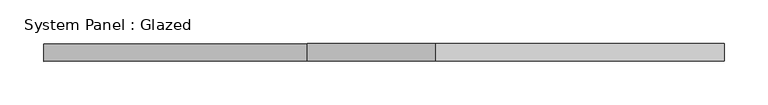
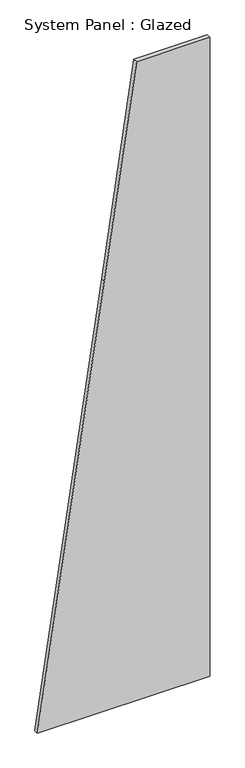
"""IFC4 building model written with IfcOpenShell, lengths in millimetres: plate geometry, System Panel : Glazed."""

import ifcopenshell
import ifcopenshell.guid

model = None  # the IFC model being written
_history = None  # IfcOwnerHistory: only IFC2X3 demands one
_inside = {}  # id of a spatial element -> (the spatial element, [elements in it])
_under = {}  # id of a project, library or spatial element -> (it, [spatial elements below it])
_declared = {}  # id of a project -> (the project, [libraries it declares])
_typed = {}  # id of a type object -> (the type object, [elements of that type])
_made_of = {}  # id of a material, layer set ... -> (it, [elements and type objects made of it])


def new_model(schema):
    """Start an empty IFC model of exactly this schema.

    Asked for "IFC4X3", IfcOpenShell would pick the latest addendum, in which some entities
    have other attributes; the version numbers below select the first issue.
    IFC2X3 requires an IfcOwnerHistory on every rooted entity: one is made here for all.
    """
    global model, _history
    if schema == "IFC4X3":
        model = ifcopenshell.file(schema_version=(4, 3, 0, 0))
    else:
        model = ifcopenshell.file(schema=schema)
    _inside.clear()
    _under.clear()
    _declared.clear()
    _typed.clear()
    _made_of.clear()
    _history = None
    if model.schema == "IFC2X3":
        org = make("IfcOrganization", Name="unknown")
        user = make(
            "IfcPersonAndOrganization",
            ThePerson=make("IfcPerson", FamilyName="unknown"),
            TheOrganization=org,
        )
        app = make(
            "IfcApplication",
            ApplicationDeveloper=org,
            Version="unknown",
            ApplicationFullName="unknown",
            ApplicationIdentifier="unknown",
        )
        _history = make(
            "IfcOwnerHistory",
            OwningUser=user,
            OwningApplication=app,
            ChangeAction="ADDED",
            CreationDate=0,
        )
    return model


def make(cls, **values):
    """One entity of the class cls with the attributes given. An attribute that is None is left unset."""
    return model.create_entity(
        cls, **{name: value for name, value in values.items() if value is not None}
    )


def rooted(cls, **values):
    """An entity with a GlobalId (a new one), such as an element, a storey or a relation."""
    return make(cls, GlobalId=ifcopenshell.guid.new(), OwnerHistory=_history, **values)


def si_unit(unit_type, name, prefix=None):
    """IfcSIUnit, for example si_unit("LENGTHUNIT", "METRE", prefix="MILLI")."""
    return make("IfcSIUnit", UnitType=unit_type, Prefix=prefix, Name=name)


def assignment(units):
    """IfcUnitAssignment: the units of a project."""
    return None if units is None else make("IfcUnitAssignment", Units=units)


def point(xyz):
    """IfcCartesianPoint."""
    return None if xyz is None else make("IfcCartesianPoint", Coordinates=xyz)


def direction(xyz):
    """IfcDirection."""
    return None if xyz is None else make("IfcDirection", DirectionRatios=xyz)


def frame(location, z_axis=None, x_axis=None):
    """IfcAxis2Placement3D, a coordinate frame: its origin and axes. An axis left out is left unset."""
    return make(
        "IfcAxis2Placement3D",
        Location=point(location),
        Axis=direction(z_axis),
        RefDirection=direction(x_axis),
    )


def origin():
    """The frame at (0, 0, 0) with its axes left unset."""
    return frame((0.0, 0.0, 0.0))


def place(relative_to, where):
    """IfcLocalPlacement: puts the frame where relative to a parent placement (None: the world)."""
    return make(
        "IfcLocalPlacement", PlacementRelTo=relative_to, RelativePlacement=where
    )


def context(
    kind, dimensions, precision=None, world=None, true_north=None, identifier=None
):
    """IfcGeometricRepresentationContext, for example the 3D "Model" context."""
    return make(
        "IfcGeometricRepresentationContext",
        ContextIdentifier=identifier,
        ContextType=kind,
        CoordinateSpaceDimension=dimensions,
        Precision=precision,
        WorldCoordinateSystem=world,
        TrueNorth=true_north,
    )


def project(units=None, contexts=None):
    """IfcProject with its units and contexts."""
    return rooted(
        "IfcProject",
        Name="project",
        RepresentationContexts=contexts,
        UnitsInContext=assignment(units),
    )


def spatial(cls, under=None, at=None, **own):
    """A site, building, storey or space (cls), placed at a placement, below another one or the project."""
    s = rooted(cls, ObjectPlacement=at, **own)
    if under is not None:
        _under.setdefault(under.id(), (under, []))[1].append(s)
    return s


def polyline(points):
    """IfcPolyline through the points."""
    return make("IfcPolyline", Points=[point(p) for p in points])


def outline(outer, holes=None, kind="AREA"):
    """IfcArbitraryClosedProfileDef: a profile drawn as a closed curve; with holes, ...WithVoids."""
    if holes is None:
        return make("IfcArbitraryClosedProfileDef", ProfileType=kind, OuterCurve=outer)
    return make(
        "IfcArbitraryProfileDefWithVoids",
        ProfileType=kind,
        OuterCurve=outer,
        InnerCurves=holes,
    )


def extrude(swept, where, along, depth):
    """IfcExtrudedAreaSolid: the profile swept, set in the frame where, extruded along a direction by depth."""
    return make(
        "IfcExtrudedAreaSolid",
        SweptArea=swept,
        Position=where,
        ExtrudedDirection=direction(along),
        Depth=depth,
    )


def shape(context_of_items, identifier, shape_type, items):
    """IfcShapeRepresentation: the items that make up one representation, for example the "Body"."""
    return make(
        "IfcShapeRepresentation",
        ContextOfItems=context_of_items,
        RepresentationIdentifier=identifier,
        RepresentationType=shape_type,
        Items=items,
    )


def source(mapping_origin, context_of_items, identifier, shape_type, items):
    """IfcRepresentationMap: a shape defined once, which mapped items show again and again."""
    return make(
        "IfcRepresentationMap",
        MappingOrigin=mapping_origin,
        MappedRepresentation=shape(context_of_items, identifier, shape_type, items),
    )


def transform(
    local_origin,
    x_axis=None,
    y_axis=None,
    z_axis=None,
    scale=None,
    scale2=None,
    scale3=None,
    uniform=True,
):
    """IfcCartesianTransformationOperator3D, or its non-uniform kind. x_axis, y_axis, z_axis: its Axis1, 2, 3."""
    if uniform:
        return make(
            "IfcCartesianTransformationOperator3D",
            Axis1=direction(x_axis),
            Axis2=direction(y_axis),
            LocalOrigin=point(local_origin),
            Scale=scale,
            Axis3=direction(z_axis),
        )
    return make(
        "IfcCartesianTransformationOperator3DnonUniform",
        Axis1=direction(x_axis),
        Axis2=direction(y_axis),
        LocalOrigin=point(local_origin),
        Scale=scale,
        Axis3=direction(z_axis),
        Scale2=scale2,
        Scale3=scale3,
    )


def mapped(mapping_source, mapping_target):
    """IfcMappedItem: shows the shape of a source again, moved by a transform."""
    return make(
        "IfcMappedItem", MappingSource=mapping_source, MappingTarget=mapping_target
    )


def made_of(thing, what):
    """Note that an element or type object is made of a material, layer set ...; save() writes the relation."""
    if what is not None:
        _made_of.setdefault(what.id(), (what, []))[1].append(thing)
    return thing


def element(
    cls,
    number,
    at=None,
    inside=None,
    cuts=None,
    type_object=None,
    material=None,
    context=None,
    identifier="Body",
    shape_type=None,
    held_by="IfcProductDefinitionShape",
    body=None,
    shapes=None,
    **own,
):
    """One element of the class cls, such as IfcWall. Its Tag is "e" and its number.

    at: its placement. inside: the storey or other place that contains it. cuts: it is an
    opening in that element (IfcRelVoidsElement). A single representation is given by context,
    identifier, shape_type and body (its items); several are given by shapes. held_by: the class
    of the entity that holds the representations. save() writes the other relations.
    """
    e = rooted(cls, Tag="e%d" % number, ObjectPlacement=at, **own)
    if body is not None:
        shapes = [shape(context, identifier, shape_type, body)]
    if shapes is not None:
        e.Representation = make(held_by, Representations=shapes)
    if inside is not None:
        _inside.setdefault(inside.id(), (inside, []))[1].append(e)
    if cuts is not None:
        rooted(
            "IfcRelVoidsElement", RelatingBuildingElement=cuts, RelatedOpeningElement=e
        )
    if type_object is not None:
        _typed.setdefault(type_object.id(), (type_object, []))[1].append(e)
    return made_of(e, material)


def aggregate(whole, parts):
    """IfcRelAggregates: a whole, such as a stair, and the parts it consists of."""
    return rooted("IfcRelAggregates", RelatingObject=whole, RelatedObjects=parts)


def save(model, path):
    """Write the relations noted so far, then the file.

    IfcRelAggregates (storeys below a building ...), IfcRelContainedInSpatialStructure (elements
    in a storey), IfcRelDefinesByType, IfcRelAssociatesMaterial and IfcRelDeclares: one each for
    every whole, place, type object, material and project.
    """
    for whole, parts in _under.values():
        aggregate(whole, parts)
    for where, things in _inside.values():
        rooted(
            "IfcRelContainedInSpatialStructure",
            RelatedElements=things,
            RelatingStructure=where,
        )
    for kind, things in _typed.values():
        rooted("IfcRelDefinesByType", RelatedObjects=things, RelatingType=kind)
    for what, things in _made_of.values():
        rooted("IfcRelAssociatesMaterial", RelatedObjects=things, RelatingMaterial=what)
    for by, libraries in _declared.values():
        rooted("IfcRelDeclares", RelatingContext=by, RelatedDefinitions=libraries)
    model.write(path)


def system_panel_glazed_f4ff012b(model_context):
    return source(origin(), model_context, "Body", "SweptSolid", [
        extrude(outline(polyline([(0.0, -389.2653129), (0.0, 389.2653129), (2060.0, 389.2653129), (3050.0, 389.2653129), (3050.0, 58.3814208), (2052.7393145, -87.9859525), (0.0, -389.2653129)])), frame((0.0, 0.0, 0.0), z_axis=(0.0, 1.0, 0.0), x_axis=(0.0, 0.0, 1.0)), (0.0, 0.0, 1.0), 20.0),
    ])


if __name__ == "__main__":
    model = new_model("IFC4")
    model_context = context("Model", 3, world=origin())
    ifc_project = project(units=[si_unit("LENGTHUNIT", "METRE", prefix="MILLI")], contexts=[model_context])
    site = spatial("IfcSite", under=ifc_project)
    building = spatial("IfcBuilding", under=site)
    placement = place(None, origin())
    system_panel_glazed_shape = system_panel_glazed_f4ff012b(model_context)
    element("IfcPlate", 1, ObjectType="System Panel : Glazed", at=placement, inside=building, context=model_context, shape_type="MappedRepresentation", body=[
        mapped(system_panel_glazed_shape, transform((0.0, 0.0, 0.0), x_axis=(1.0, 0.0, 0.0), y_axis=(0.0, 1.0, 0.0), z_axis=(0.0, 0.0, 1.0))),
    ])
    save(model, "model.ifc")

# Revit data of these elements
# Type "System Panel : Glazed"
#   COBie.Type = no
# Element 1 (IfcPlate, "System Panel : Glazed")
#   Materials on its faces: "Glass"
# Materials
#   "Glass": class "Glass", colour RGB 0 128 192, transparency 0.75, Description = "Soda Lime Glass", Cost = 0
